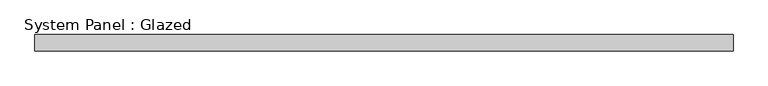
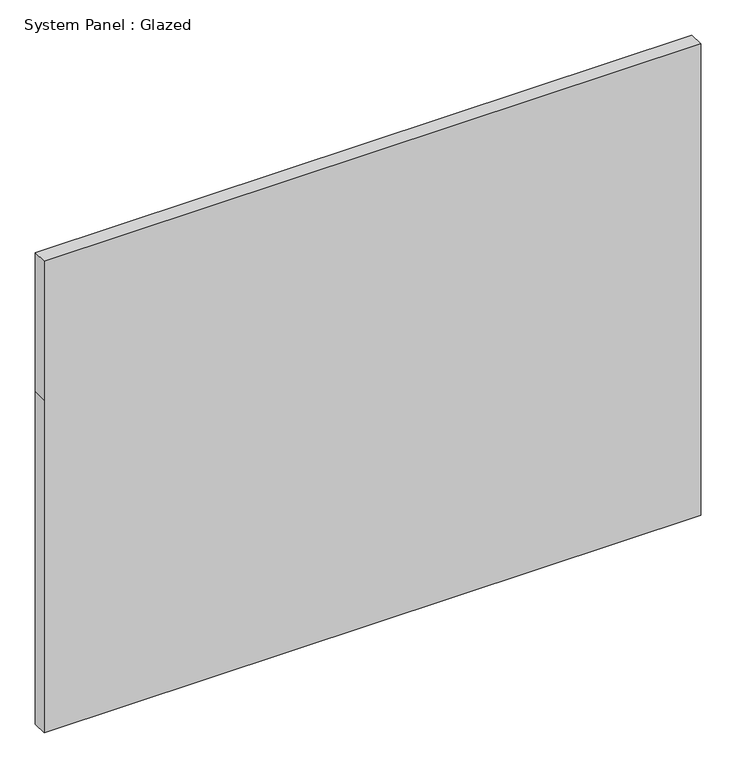
"""IFC4 building model written with IfcOpenShell, lengths in millimetres: plate geometry, System Panel : Glazed."""

from ifc_helpers import new_model, si_unit, frame, origin, place, context, project, spatial, polyline, outline, extrude, source, transform, mapped, element, save


def system_panel_glazed_a8813c32(model_context):
    return source(origin(), model_context, "Body", "SweptSolid", [
        extrude(outline(polyline([(0.0, -539.5993644), (0.0, 539.5993644), (577.85, 539.5993644), (819.15, 539.5993644), (819.15, -539.5993644), (577.85, -539.5993644), (0.0, -539.5993644)])), frame((0.0, -44.45, 0.0), z_axis=(0.0, 1.0, 0.0), x_axis=(0.0, 0.0, 1.0)), (0.0, 0.0, 1.0), 25.4),
    ])


if __name__ == "__main__":
    model = new_model("IFC4")
    model_context = context("Model", 3, world=origin())
    ifc_project = project(units=[si_unit("LENGTHUNIT", "METRE", prefix="MILLI")], contexts=[model_context])
    site = spatial("IfcSite", under=ifc_project)
    building = spatial("IfcBuilding", under=site)
    placement = place(None, origin())
    system_panel_glazed_shape = system_panel_glazed_a8813c32(model_context)
    element("IfcPlate", 1, ObjectType="System Panel : Glazed", at=placement, inside=building, context=model_context, shape_type="MappedRepresentation", body=[
        mapped(system_panel_glazed_shape, transform((0.0, 0.0, 0.0), x_axis=(1.0, 0.0, 0.0), y_axis=(0.0, 1.0, 0.0), z_axis=(0.0, 0.0, 1.0))),
    ])
    save(model, "model.ifc")

# Revit data of these elements
# Element 1 (IfcPlate, "System Panel : Glazed")
#   Materials on its faces: "Glass"
# Materials
#   "Glass": class "Unassigned", colour RGB 147 173 200, transparency 0.7, Cost = 0
